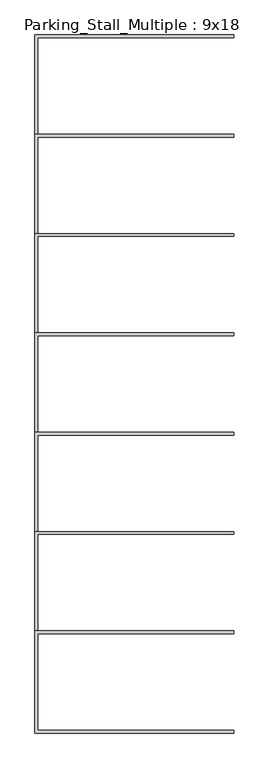
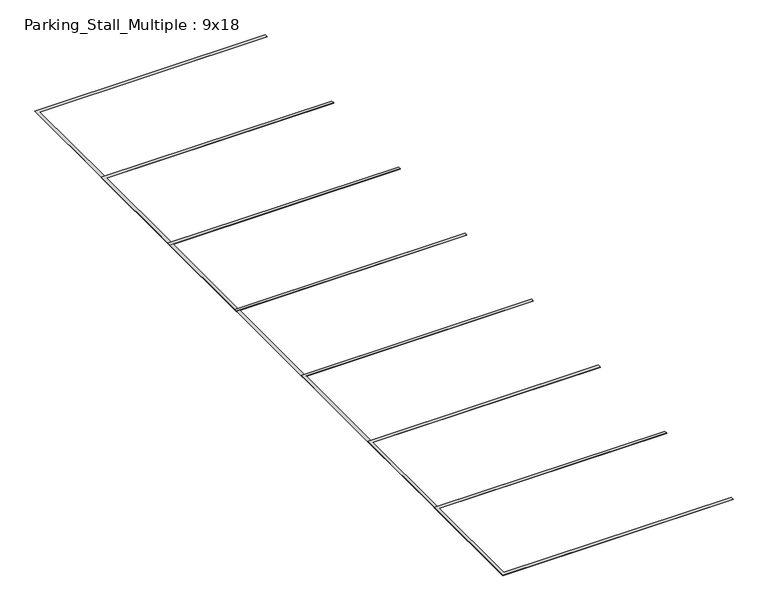
"""IFC4 building model written with IfcOpenShell, lengths in millimetres: proxy geometry, Parking_Stall_Multiple : 9x18."""

from ifc_helpers import new_model, si_unit, origin, origin_with_axes, place, context, project, spatial, polyline, outline, extrude, source, transform, mapped, element, save


def parking_stall_multiple_9x18_f9c0f0b0(model_context):
    return source(origin(), model_context, "Body", "SweptSolid", [
        extrude(outline(polyline([(5486.4, -16459.2), (5486.4, -16535.4), (76.2, -16535.4), (76.2, -19202.4), (5486.4, -19202.4), (5486.4, -19278.6), (0.0, -19278.6), (0.0, -16459.2), (5486.4, -16459.2)])), origin_with_axes(), (0.0, 0.0, 1.0), 6.35),
        extrude(outline(polyline([(5486.4, -13716.0), (5486.4, -13792.2), (76.2, -13792.2), (76.2, -16459.2), (5486.4, -16459.2), (5486.4, -16535.4), (0.0, -16535.4), (0.0, -13716.0), (5486.4, -13716.0)])), origin_with_axes(), (0.0, 0.0, 1.0), 6.35),
        extrude(outline(polyline([(5486.4, -10972.8), (5486.4, -11049.0), (76.2, -11049.0), (76.2, -13716.0), (5486.4, -13716.0), (5486.4, -13792.2), (0.0, -13792.2), (0.0, -10972.8), (5486.4, -10972.8)])), origin_with_axes(), (0.0, 0.0, 1.0), 6.35),
        extrude(outline(polyline([(5486.4, -8229.6), (5486.4, -8305.8), (76.2, -8305.8), (76.2, -10972.8), (5486.4, -10972.8), (5486.4, -11049.0), (0.0, -11049.0), (0.0, -8229.6), (5486.4, -8229.6)])), origin_with_axes(), (0.0, 0.0, 1.0), 6.35),
        extrude(outline(polyline([(5486.4, -5486.4), (5486.4, -5562.6), (76.2, -5562.6), (76.2, -8229.6), (5486.4, -8229.6), (5486.4, -8305.8), (0.0, -8305.8), (0.0, -5486.4), (5486.4, -5486.4)])), origin_with_axes(), (0.0, 0.0, 1.0), 6.35),
        extrude(outline(polyline([(5486.4, -2743.2), (5486.4, -2819.4), (76.2, -2819.4), (76.2, -5486.4), (5486.4, -5486.4), (5486.4, -5562.6), (0.0, -5562.6), (0.0, -2743.2), (5486.4, -2743.2)])), origin_with_axes(), (0.0, 0.0, 1.0), 6.35),
        extrude(outline(polyline([(5486.4, 0.0), (5486.4, -76.2), (76.2, -76.2), (76.2, -2743.2), (5486.4, -2743.2), (5486.4, -2819.4), (0.0, -2819.4), (0.0, 0.0), (5486.4, 0.0)])), origin_with_axes(), (0.0, 0.0, 1.0), 6.35),
    ])


if __name__ == "__main__":
    model = new_model("IFC4")
    model_context = context("Model", 3, world=origin())
    ifc_project = project(units=[si_unit("LENGTHUNIT", "METRE", prefix="MILLI")], contexts=[model_context])
    site = spatial("IfcSite", under=ifc_project)
    building = spatial("IfcBuilding", under=site)
    placement = place(None, origin())
    parking_stall_multiple_9x18_shape = parking_stall_multiple_9x18_f9c0f0b0(model_context)
    element("IfcBuildingElementProxy", 1, Name="Parking_Stall_Multiple : 9x18", ObjectType="Parking_Stall_Multiple : 9x18", at=placement, inside=building, context=model_context, shape_type="MappedRepresentation", body=[
        mapped(parking_stall_multiple_9x18_shape, transform((0.0, 0.0, 0.0), x_axis=(1.0, 0.0, 0.0), y_axis=(0.0, 1.0, 0.0), z_axis=(0.0, 0.0, 1.0))),
    ])
    save(model, "model.ifc")

# Revit data of these elements
# Type "Parking_Stall_Multiple : 9x18"
#   Parking_Width_M = 9' - 0"
#   Parking_Run_Length [instance default] = 65' - 0"
#   Parking_Line_Width = 0' - 3"
#   Parking_Length_M = 18' - 0"
#   Single_Parking_Visibility [instance default] = no
#   Parking_ADA_Symbol = no
#   ParkingUnitsArray [instance default] = 7
#   ParkingUnits [instance default] = 7
#   Multiple_Parking_Visibility [instance default] = yes
#   Parking_Line_Material = ADA VAN ACCESSIBLE STALL
# Element 1 (IfcBuildingElementProxy, "Parking_Stall_Multiple : 9x18")
#   Parking_Run_Length = 60' - 11.70354"
#   Materials on its faces: "ADA VAN ACCESSIBLE STALL"
# Materials
#   "ADA VAN ACCESSIBLE STALL": class "Paint", colour RGB 255 255 255, transparency 0, Cost = 0
